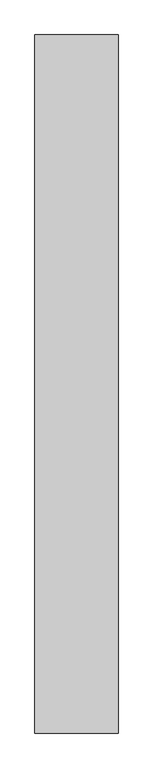
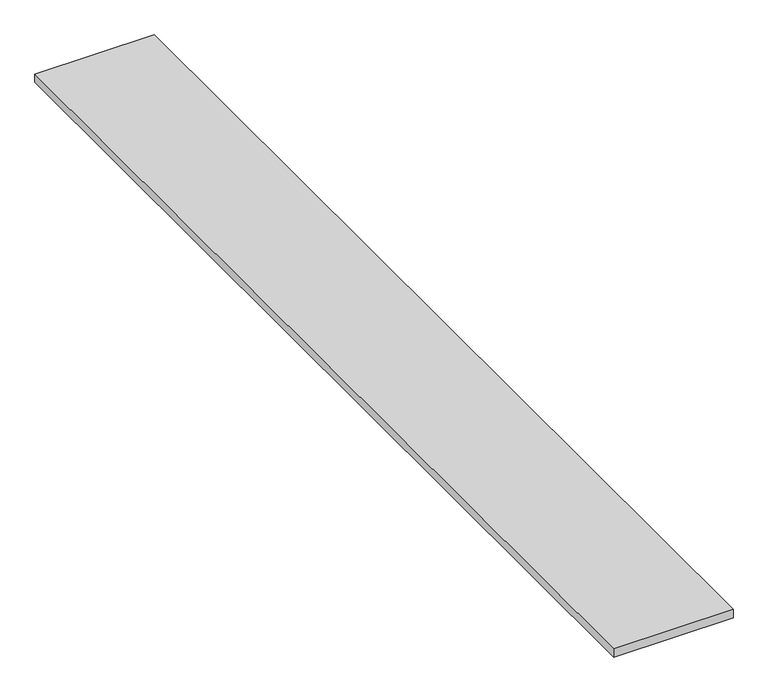
"""IFC4 building model written with IfcOpenShell, lengths in millimetres: furniture geometry, Furniture 3:Furniture 1:2413:Furniture 1:2413 : Furniture 3:Furniture 1:2413:300430 : Furniture 3:Furniture 1:2413:Furniture 1:2413 : Furniture 3:Furniture 1:2413:300430."""

from ifc_helpers import new_model, si_unit, frame, origin, place, context, project, spatial, polyline, outline, extrude, source, transform, mapped, element, save


def furniture_44db3b27(model_context):
    return source(origin(), model_context, "Body", "SweptSolid", [
        extrude(outline(polyline([(644560.3117239, -575267.6690318), (644204.7117239, -575267.6690318), (644204.7117239, -572280.41257), (644560.3117239, -572280.41257), (644560.3117239, -575267.6690318)])), frame((0.0, 0.0, 381.0), z_axis=(0.0, 0.0, 1.0), x_axis=(1.0, 0.0, 0.0)), (0.0, 0.0, 1.0), 25.4),
    ])


if __name__ == "__main__":
    model = new_model("IFC4")
    model_context = context("Model", 3, world=origin())
    ifc_project = project(units=[si_unit("LENGTHUNIT", "METRE", prefix="MILLI")], contexts=[model_context])
    site = spatial("IfcSite", under=ifc_project)
    building = spatial("IfcBuilding", under=site)
    placement = place(None, origin())
    furniture_shape = furniture_44db3b27(model_context)
    element("IfcFurniture", 1, ObjectType="Furniture 3:Furniture 1:2413:Furniture 1:2413 : Furniture 3:Furniture 1:2413:300430 : Furniture 3:Furniture 1:2413:Furniture 1:2413 : Furniture 3:Furniture 1:2413:300430", at=placement, inside=building, context=model_context, shape_type="MappedRepresentation", body=[
        mapped(furniture_shape, transform((0.0, 0.0, 0.0), x_axis=(1.0, 0.0, 0.0), y_axis=(0.0, 1.0, 0.0), z_axis=(0.0, 0.0, 1.0))),
    ])
    save(model, "model.ifc")

# Revit data of these elements
# Type "Furniture 3:Furniture 1:2413:Furniture 1:2413 : Furniture 3:Furniture 1:2413:300430 : Furniture 3:Furniture 1:2413:Furniture 1:2413 : Furniture 3:Furniture 1:2413:300430"
#   NameOverride = "Furniture 3:Furniture 1:2413:Furniture 1:2413 : Furniture 3:Furniture 1:2413:300430"
#   ObjectTypeOverride = "Furniture 1:2413 : Furniture 3:Furniture 1:2413"
#   Tag = "300430"
